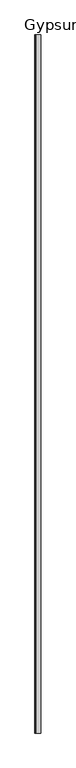
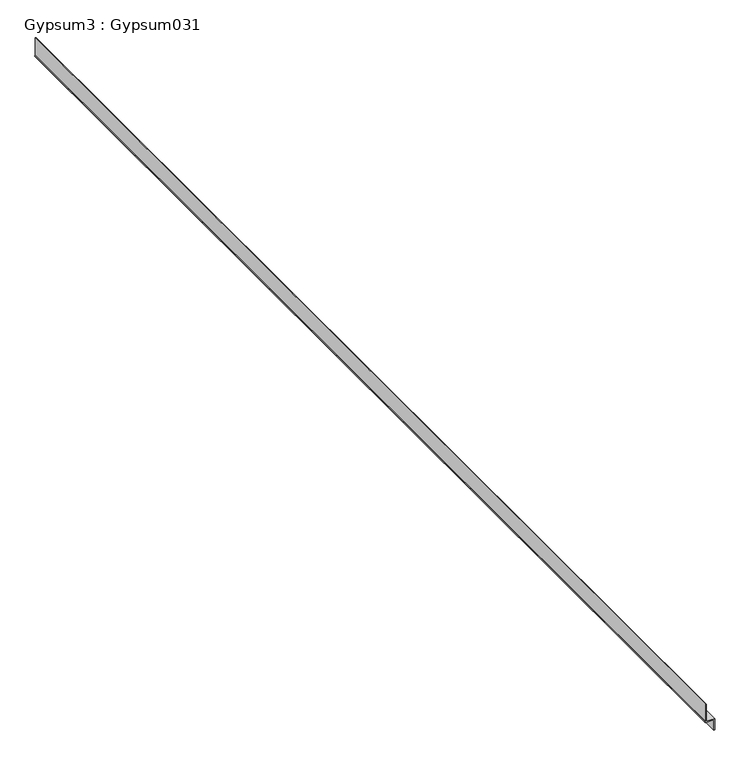
"""IFC4 building model written with IfcOpenShell, lengths in millimetres: proxy geometry, Gypsum3 : Gypsum031."""

import ifcopenshell
import ifcopenshell.guid

model = None  # the IFC model being written
_history = None  # IfcOwnerHistory: only IFC2X3 demands one
_inside = {}  # id of a spatial element -> (the spatial element, [elements in it])
_under = {}  # id of a project, library or spatial element -> (it, [spatial elements below it])
_declared = {}  # id of a project -> (the project, [libraries it declares])
_typed = {}  # id of a type object -> (the type object, [elements of that type])
_made_of = {}  # id of a material, layer set ... -> (it, [elements and type objects made of it])


def new_model(schema):
    """Start an empty IFC model of exactly this schema.

    Asked for "IFC4X3", IfcOpenShell would pick the latest addendum, in which some entities
    have other attributes; the version numbers below select the first issue.
    IFC2X3 requires an IfcOwnerHistory on every rooted entity: one is made here for all.
    """
    global model, _history
    if schema == "IFC4X3":
        model = ifcopenshell.file(schema_version=(4, 3, 0, 0))
    else:
        model = ifcopenshell.file(schema=schema)
    _inside.clear()
    _under.clear()
    _declared.clear()
    _typed.clear()
    _made_of.clear()
    _history = None
    if model.schema == "IFC2X3":
        org = make("IfcOrganization", Name="unknown")
        user = make(
            "IfcPersonAndOrganization",
            ThePerson=make("IfcPerson", FamilyName="unknown"),
            TheOrganization=org,
        )
        app = make(
            "IfcApplication",
            ApplicationDeveloper=org,
            Version="unknown",
            ApplicationFullName="unknown",
            ApplicationIdentifier="unknown",
        )
        _history = make(
            "IfcOwnerHistory",
            OwningUser=user,
            OwningApplication=app,
            ChangeAction="ADDED",
            CreationDate=0,
        )
    return model


def make(cls, **values):
    """One entity of the class cls with the attributes given. An attribute that is None is left unset."""
    return model.create_entity(
        cls, **{name: value for name, value in values.items() if value is not None}
    )


def rooted(cls, **values):
    """An entity with a GlobalId (a new one), such as an element, a storey or a relation."""
    return make(cls, GlobalId=ifcopenshell.guid.new(), OwnerHistory=_history, **values)


def si_unit(unit_type, name, prefix=None):
    """IfcSIUnit, for example si_unit("LENGTHUNIT", "METRE", prefix="MILLI")."""
    return make("IfcSIUnit", UnitType=unit_type, Prefix=prefix, Name=name)


def assignment(units):
    """IfcUnitAssignment: the units of a project."""
    return None if units is None else make("IfcUnitAssignment", Units=units)


def point(xyz):
    """IfcCartesianPoint."""
    return None if xyz is None else make("IfcCartesianPoint", Coordinates=xyz)


def direction(xyz):
    """IfcDirection."""
    return None if xyz is None else make("IfcDirection", DirectionRatios=xyz)


def frame(location, z_axis=None, x_axis=None):
    """IfcAxis2Placement3D, a coordinate frame: its origin and axes. An axis left out is left unset."""
    return make(
        "IfcAxis2Placement3D",
        Location=point(location),
        Axis=direction(z_axis),
        RefDirection=direction(x_axis),
    )


def origin():
    """The frame at (0, 0, 0) with its axes left unset."""
    return frame((0.0, 0.0, 0.0))


def place(relative_to, where):
    """IfcLocalPlacement: puts the frame where relative to a parent placement (None: the world)."""
    return make(
        "IfcLocalPlacement", PlacementRelTo=relative_to, RelativePlacement=where
    )


def context(
    kind, dimensions, precision=None, world=None, true_north=None, identifier=None
):
    """IfcGeometricRepresentationContext, for example the 3D "Model" context."""
    return make(
        "IfcGeometricRepresentationContext",
        ContextIdentifier=identifier,
        ContextType=kind,
        CoordinateSpaceDimension=dimensions,
        Precision=precision,
        WorldCoordinateSystem=world,
        TrueNorth=true_north,
    )


def project(units=None, contexts=None):
    """IfcProject with its units and contexts."""
    return rooted(
        "IfcProject",
        Name="project",
        RepresentationContexts=contexts,
        UnitsInContext=assignment(units),
    )


def spatial(cls, under=None, at=None, **own):
    """A site, building, storey or space (cls), placed at a placement, below another one or the project."""
    s = rooted(cls, ObjectPlacement=at, **own)
    if under is not None:
        _under.setdefault(under.id(), (under, []))[1].append(s)
    return s


def polyline(points):
    """IfcPolyline through the points."""
    return make("IfcPolyline", Points=[point(p) for p in points])


def outline(outer, holes=None, kind="AREA"):
    """IfcArbitraryClosedProfileDef: a profile drawn as a closed curve; with holes, ...WithVoids."""
    if holes is None:
        return make("IfcArbitraryClosedProfileDef", ProfileType=kind, OuterCurve=outer)
    return make(
        "IfcArbitraryProfileDefWithVoids",
        ProfileType=kind,
        OuterCurve=outer,
        InnerCurves=holes,
    )


def extrude(swept, where, along, depth):
    """IfcExtrudedAreaSolid: the profile swept, set in the frame where, extruded along a direction by depth."""
    return make(
        "IfcExtrudedAreaSolid",
        SweptArea=swept,
        Position=where,
        ExtrudedDirection=direction(along),
        Depth=depth,
    )


def shape(context_of_items, identifier, shape_type, items):
    """IfcShapeRepresentation: the items that make up one representation, for example the "Body"."""
    return make(
        "IfcShapeRepresentation",
        ContextOfItems=context_of_items,
        RepresentationIdentifier=identifier,
        RepresentationType=shape_type,
        Items=items,
    )


def source(mapping_origin, context_of_items, identifier, shape_type, items):
    """IfcRepresentationMap: a shape defined once, which mapped items show again and again."""
    return make(
        "IfcRepresentationMap",
        MappingOrigin=mapping_origin,
        MappedRepresentation=shape(context_of_items, identifier, shape_type, items),
    )


def transform(
    local_origin,
    x_axis=None,
    y_axis=None,
    z_axis=None,
    scale=None,
    scale2=None,
    scale3=None,
    uniform=True,
):
    """IfcCartesianTransformationOperator3D, or its non-uniform kind. x_axis, y_axis, z_axis: its Axis1, 2, 3."""
    if uniform:
        return make(
            "IfcCartesianTransformationOperator3D",
            Axis1=direction(x_axis),
            Axis2=direction(y_axis),
            LocalOrigin=point(local_origin),
            Scale=scale,
            Axis3=direction(z_axis),
        )
    return make(
        "IfcCartesianTransformationOperator3DnonUniform",
        Axis1=direction(x_axis),
        Axis2=direction(y_axis),
        LocalOrigin=point(local_origin),
        Scale=scale,
        Axis3=direction(z_axis),
        Scale2=scale2,
        Scale3=scale3,
    )


def mapped(mapping_source, mapping_target):
    """IfcMappedItem: shows the shape of a source again, moved by a transform."""
    return make(
        "IfcMappedItem", MappingSource=mapping_source, MappingTarget=mapping_target
    )


def made_of(thing, what):
    """Note that an element or type object is made of a material, layer set ...; save() writes the relation."""
    if what is not None:
        _made_of.setdefault(what.id(), (what, []))[1].append(thing)
    return thing


def element(
    cls,
    number,
    at=None,
    inside=None,
    cuts=None,
    type_object=None,
    material=None,
    context=None,
    identifier="Body",
    shape_type=None,
    held_by="IfcProductDefinitionShape",
    body=None,
    shapes=None,
    **own,
):
    """One element of the class cls, such as IfcWall. Its Tag is "e" and its number.

    at: its placement. inside: the storey or other place that contains it. cuts: it is an
    opening in that element (IfcRelVoidsElement). A single representation is given by context,
    identifier, shape_type and body (its items); several are given by shapes. held_by: the class
    of the entity that holds the representations. save() writes the other relations.
    """
    e = rooted(cls, Tag="e%d" % number, ObjectPlacement=at, **own)
    if body is not None:
        shapes = [shape(context, identifier, shape_type, body)]
    if shapes is not None:
        e.Representation = make(held_by, Representations=shapes)
    if inside is not None:
        _inside.setdefault(inside.id(), (inside, []))[1].append(e)
    if cuts is not None:
        rooted(
            "IfcRelVoidsElement", RelatingBuildingElement=cuts, RelatedOpeningElement=e
        )
    if type_object is not None:
        _typed.setdefault(type_object.id(), (type_object, []))[1].append(e)
    return made_of(e, material)


def aggregate(whole, parts):
    """IfcRelAggregates: a whole, such as a stair, and the parts it consists of."""
    return rooted("IfcRelAggregates", RelatingObject=whole, RelatedObjects=parts)


def save(model, path):
    """Write the relations noted so far, then the file.

    IfcRelAggregates (storeys below a building ...), IfcRelContainedInSpatialStructure (elements
    in a storey), IfcRelDefinesByType, IfcRelAssociatesMaterial and IfcRelDeclares: one each for
    every whole, place, type object, material and project.
    """
    for whole, parts in _under.values():
        aggregate(whole, parts)
    for where, things in _inside.values():
        rooted(
            "IfcRelContainedInSpatialStructure",
            RelatedElements=things,
            RelatingStructure=where,
        )
    for kind, things in _typed.values():
        rooted("IfcRelDefinesByType", RelatedObjects=things, RelatingType=kind)
    for what, things in _made_of.values():
        rooted("IfcRelAssociatesMaterial", RelatedObjects=things, RelatingMaterial=what)
    for by, libraries in _declared.values():
        rooted("IfcRelDeclares", RelatingContext=by, RelatedDefinitions=libraries)
    model.write(path)


def gypsum3_gypsum031_486e7f05(model_context):
    return source(origin(), model_context, "Body", "SweptSolid", [
        extrude(outline(polyline([(40163.496, 16336.5357412), (40163.496, 16337.8057412), (40183.866, 16337.8057412), (40183.866, 16323.5175016), (40215.616, 16323.5175016), (40215.616, 16322.2475016), (40183.866, 16322.2475016), (40183.866, 16321.4376545), (40182.596, 16321.4376545), (40182.596, 16336.5357412), (40163.496, 16336.5357412)])), frame((0.0, -1052.8906567, 0.0), z_axis=(0.0, 1.0, 0.0), x_axis=(0.0, 0.0, 1.0)), (0.0, 0.0, 1.0), 1999.85),
    ])


if __name__ == "__main__":
    model = new_model("IFC4")
    model_context = context("Model", 3, world=origin())
    ifc_project = project(units=[si_unit("LENGTHUNIT", "METRE", prefix="MILLI")], contexts=[model_context])
    site = spatial("IfcSite", under=ifc_project)
    building = spatial("IfcBuilding", under=site)
    placement = place(None, origin())
    gypsum3_gypsum031_shape = gypsum3_gypsum031_486e7f05(model_context)
    element("IfcBuildingElementProxy", 1, Name="Gypsum3 : Gypsum031", ObjectType="Gypsum3 : Gypsum031", at=placement, inside=building, context=model_context, shape_type="MappedRepresentation", body=[
        mapped(gypsum3_gypsum031_shape, transform((0.0, 0.0, 0.0), x_axis=(1.0, 0.0, 0.0), y_axis=(0.0, 1.0, 0.0), z_axis=(0.0, 0.0, 1.0))),
    ])
    save(model, "model.ifc")

# Revit data of these elements
# Type "Gypsum3 : Gypsum031"
#   NameOverride = "Gypsum031"
# Element 1 (IfcBuildingElementProxy, "Gypsum3 : Gypsum031")
#   Materials on its faces: "SHADOW Z REVEAL  BEAD"
# Materials
#   "SHADOW Z REVEAL  BEAD": class "Unassigned", colour RGB 251 232 155, transparency 0, Cost = 0
